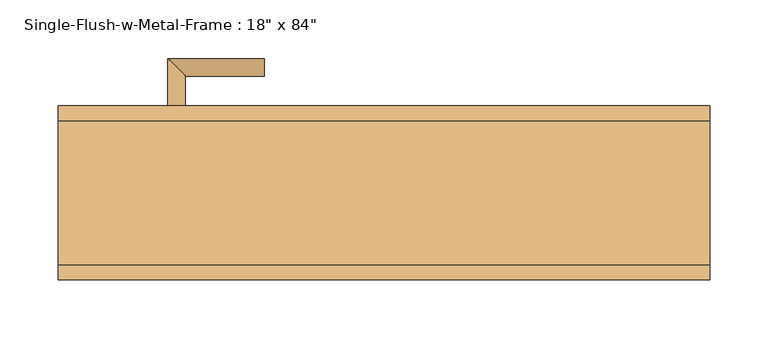
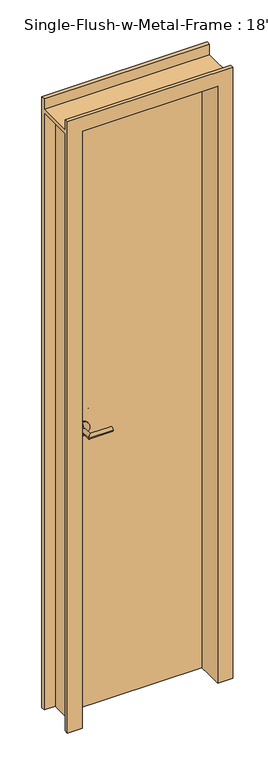
"""IFC4 building model written with IfcOpenShell, lengths in millimetres: door geometry."""

from ifc_helpers import new_model, si_unit, point, frame, origin, origin_with_axes, place, context, project, spatial, polyline, circle_curve, ellipse_curve, trimmed, outline, extrude, faceted_brep, source, transform, mapped, element, save
from ifc_brep_helpers import plane_surface, cylinder_surface, revolved_surface, advanced_brep


def door_d799fe97(model_context):
    return source(origin(), model_context, "Body", "SolidModel", [
        advanced_brep(
        [(-177.8, 14.2875, 971.55), (-177.8, 5.7988821, 989.45), (-185.3, 5.7988821, 996.95), (-177.8, 5.7988821, 1004.45), (-177.8, 14.2875, 1022.35), (-170.3, 5.7988821, 996.95), (-177.8, 17.4625, 1022.35), (-177.8, 17.4625, 971.55), (-177.8, 17.4625, 996.95), (-185.3, -36.1375, 996.95), (-170.3, -21.1375, 996.95), (-102.8, -36.1375, 996.95), (-102.8, -21.1375, 996.95)],
        [
            (0, 1, circle_curve(frame((-177.8, -22.3167775, 965.1541113), z_axis=(1.0, 0.0, 0.0), x_axis=(0.0, 0.0, 1.0)), 37.1588553)),
            (1, 2, circle_curve(frame((-177.8, 5.7988821, 996.95), z_axis=(0.0, 1.0, 0.0), x_axis=(0.0, 0.0, 1.0)), 7.5)),
            (2, 3, circle_curve(frame((-177.8, 5.7988821, 996.95), z_axis=(0.0, 1.0, 0.0), x_axis=(0.0, 0.0, 1.0)), 7.5)),
            (3, 4, circle_curve(frame((-177.8, -22.3167775, 1028.7458887), z_axis=(1.0, 0.0, 0.0), x_axis=(0.0, 0.0, -1.0)), 37.1588553)),
            (4, 0, circle_curve(frame((-177.8, 14.2875, 996.95), z_axis=(0.0, -1.0, 0.0), x_axis=(0.0, 0.0, 1.0)), 25.4)),
            (3, 5, circle_curve(frame((-177.8, 5.7988821, 996.95), z_axis=(0.0, 1.0, 0.0), x_axis=(0.0, 0.0, 1.0)), 7.5)),
            (5, 1, circle_curve(frame((-177.8, 5.7988821, 996.95), z_axis=(0.0, 1.0, 0.0), x_axis=(0.0, 0.0, 1.0)), 7.5)),
            (0, 4, circle_curve(frame((-177.8, 14.2875, 996.95), z_axis=(0.0, -1.0, 0.0), x_axis=(0.0, 0.0, 1.0)), 25.4)),
            (4, 6),
            (6, 7, circle_curve(frame((-177.8, 17.4625, 996.95), z_axis=(0.0, -1.0, 0.0), x_axis=(0.0, 0.0, 1.0)), 25.4)),
            (7, 0),
            (7, 6, circle_curve(frame((-177.8, 17.4625, 996.95), z_axis=(0.0, -1.0, 0.0), x_axis=(0.0, 0.0, 1.0)), 25.4)),
            (6, 8),
            (8, 7),
            (9, 2),
            (5, 10),
            (10, 9, ellipse_curve(frame((-177.8, -28.6375, 996.95), z_axis=(-0.7071067811864695, 0.7071067811866254, 0.0), x_axis=(0.7071067811866254, 0.7071067811864696, 0.0)), 10.6066017, 7.5)),
            (9, 10, ellipse_curve(frame((-177.8, -28.6375, 996.95), z_axis=(-0.7071067811864695, 0.7071067811866254, 0.0), x_axis=(0.7071067811866254, 0.7071067811864696, 0.0)), 10.6066017, 7.5)),
            (11, 12, circle_curve(frame((-102.8, -28.6375, 996.95), z_axis=(1.0, 0.0, 0.0), x_axis=(0.0, 1.0, 0.0)), 7.5)),
            (12, 11, circle_curve(frame((-102.8, -28.6375, 996.95), z_axis=(1.0, 0.0, 0.0), x_axis=(0.0, 1.0, 0.0)), 7.5)),
            (10, 12),
            (11, 9),
        ],
        [
            revolved_surface(trimmed(ellipse_curve(frame((-177.8, -22.3167775, 1028.7458887), z_axis=(1.0, 0.0, 0.0), x_axis=(0.0, 0.0, -1.0)), 37.1588553, 37.1588553), [point((-177.8, 4.7625, 1003.3))], [point((-177.8, 14.2875, 1022.35))], True, "CARTESIAN"), (-177.8, 4.7625, 996.95), (0.0, 1.0, 0.0)),
            cylinder_surface(frame((-177.8, 4.7625, 996.95), z_axis=(0.0, 1.0, 0.0), x_axis=(0.0, 0.0, 1.0)), 25.4),
            plane_surface(frame((-177.8, 17.4625, 996.95), z_axis=(0.0, 1.0, 0.0), x_axis=(0.0, 0.0, 1.0))),
            cylinder_surface(frame((-177.8, 9.4625, 996.95), z_axis=(0.0, 1.0, 0.0), x_axis=(1.0, 0.0, 0.0)), 7.5),
            plane_surface(frame((-102.8, -28.6375, 996.95), z_axis=(1.0, 0.0, 0.0), x_axis=(0.0, 0.0, 1.0))),
            cylinder_surface(frame((-177.8, -28.6375, 996.95), z_axis=(-1.0, 0.0, 0.0), x_axis=(0.0, 1.0, 0.0)), 7.5),
        ],
        [
            (0, [[1, 2, 3, 4, 5]]),
            (0, [[-4, 6, 7, -1, 8]]),
            (1, [[9, 10, 11, -5]]),
            (1, [[-11, 12, -9, -8]]),
            (2, [[13, 14, -10]]),
            (2, [[-14, -13, -12]]),
            (3, [[15, -2, -7, 16, 17]]),
            (3, [[-16, -6, -3, -15, 18]]),
            (4, [[19, 20]]),
            (5, [[21, -19, 22, -17]]),
            (5, [[-22, -20, -21, -18]]),
        ],
    ),
        advanced_brep(
        [(-177.8, 65.0875, 971.55), (-177.8, 65.0875, 1022.35), (-177.8, 73.5761179, 1004.45), (-185.3, 73.5761179, 996.95), (-177.8, 73.5761179, 989.45), (-170.3, 73.5761179, 996.95), (-177.8, 61.9125, 971.55), (-177.8, 61.9125, 1022.35), (-177.8, 61.9125, 996.95), (-185.3, 115.5125, 996.95), (-170.3, 100.5125, 996.95), (-102.8, 115.5125, 996.95), (-102.8, 100.5125, 996.95)],
        [
            (0, 1, circle_curve(frame((-177.8, 65.0875, 996.95), z_axis=(0.0, 1.0, 0.0), x_axis=(0.0, 0.0, 1.0)), 25.4)),
            (1, 2, circle_curve(frame((-177.8, 101.6917775, 1028.7458887), z_axis=(1.0, 0.0, 0.0), x_axis=(0.0, 0.0, -1.0)), 37.1588553)),
            (2, 3, circle_curve(frame((-177.8, 73.5761179, 996.95), z_axis=(0.0, -1.0, 0.0), x_axis=(0.0, 0.0, 1.0)), 7.5)),
            (3, 4, circle_curve(frame((-177.8, 73.5761179, 996.95), z_axis=(0.0, -1.0, 0.0), x_axis=(0.0, 0.0, 1.0)), 7.5)),
            (4, 0, circle_curve(frame((-177.8, 101.6917775, 965.1541113), z_axis=(1.0, 0.0, 0.0), x_axis=(0.0, 0.0, 1.0)), 37.1588553)),
            (1, 0, circle_curve(frame((-177.8, 65.0875, 996.95), z_axis=(0.0, 1.0, 0.0), x_axis=(0.0, 0.0, 1.0)), 25.4)),
            (4, 5, circle_curve(frame((-177.8, 73.5761179, 996.95), z_axis=(0.0, -1.0, 0.0), x_axis=(0.0, 0.0, 1.0)), 7.5)),
            (5, 2, circle_curve(frame((-177.8, 73.5761179, 996.95), z_axis=(0.0, -1.0, 0.0), x_axis=(0.0, 0.0, 1.0)), 7.5)),
            (0, 6),
            (6, 7, circle_curve(frame((-177.8, 61.9125, 996.95), z_axis=(0.0, 1.0, 0.0), x_axis=(0.0, 0.0, 1.0)), 25.4)),
            (7, 1),
            (7, 6, circle_curve(frame((-177.8, 61.9125, 996.95), z_axis=(0.0, 1.0, 0.0), x_axis=(0.0, 0.0, 1.0)), 25.4)),
            (6, 8),
            (8, 7),
            (9, 10, ellipse_curve(frame((-177.8, 108.0125, 996.95), z_axis=(-0.7071067811864695, -0.7071067811866254, 0.0), x_axis=(0.7071067811866254, -0.7071067811864696, 0.0)), 10.6066017, 7.5)),
            (10, 5),
            (3, 9),
            (10, 9, ellipse_curve(frame((-177.8, 108.0125, 996.95), z_axis=(-0.7071067811864695, -0.7071067811866254, 0.0), x_axis=(0.7071067811866254, -0.7071067811864696, 0.0)), 10.6066017, 7.5)),
            (11, 12, circle_curve(frame((-102.8, 108.0125, 996.95), z_axis=(1.0, 0.0, 0.0), x_axis=(0.0, -1.0, 0.0)), 7.5)),
            (12, 11, circle_curve(frame((-102.8, 108.0125, 996.95), z_axis=(1.0, 0.0, 0.0), x_axis=(0.0, -1.0, 0.0)), 7.5)),
            (9, 11),
            (12, 10),
        ],
        [
            revolved_surface(trimmed(ellipse_curve(frame((-177.8, 101.6917775, 1028.7458887), z_axis=(-1.0, 0.0, 0.0), x_axis=(0.0, 0.0, -1.0)), 37.1588553, 37.1588553), [point((-177.8, 74.6125, 1003.3))], [point((-177.8, 65.0875, 1022.35))], True, "CARTESIAN"), (-177.8, 74.6125, 996.95), (0.0, -1.0, 0.0)),
            cylinder_surface(frame((-177.8, 74.6125, 996.95), z_axis=(0.0, -1.0, 0.0), x_axis=(0.0, 0.0, 1.0)), 25.4),
            plane_surface(frame((-177.8, 61.9125, 996.95), z_axis=(0.0, -1.0, 0.0), x_axis=(0.0, 0.0, 1.0))),
            cylinder_surface(frame((-177.8, 69.9125, 996.95), z_axis=(0.0, -1.0, 0.0), x_axis=(1.0, 0.0, 0.0)), 7.5),
            plane_surface(frame((-102.8, 108.0125, 996.95), z_axis=(1.0, 0.0, 0.0), x_axis=(0.0, 0.0, 1.0))),
            cylinder_surface(frame((-177.8, 108.0125, 996.95), z_axis=(-1.0, 0.0, 0.0), x_axis=(0.0, -1.0, 0.0)), 7.5),
        ],
        [
            (0, [[1, 2, 3, 4, 5]]),
            (0, [[6, -5, 7, 8, -2]]),
            (1, [[-1, 9, 10, 11]]),
            (1, [[-6, -11, 12, -9]]),
            (2, [[-10, 13, 14]]),
            (2, [[-12, -14, -13]]),
            (3, [[15, 16, -7, -4, 17]]),
            (3, [[18, -17, -3, -8, -16]]),
            (4, [[19, 20]]),
            (5, [[-15, 21, -20, 22]]),
            (5, [[-18, -22, -19, -21]]),
        ],
    ),
        extrude(outline(polyline([(228.6, 17.4625), (-228.6, 17.4625), (-228.6, 61.9125), (228.6, 61.9125), (228.6, 17.4625)])), origin_with_axes(), (0.0, 0.0, 1.0), 2133.6),
        faceted_brep([(-241.3, 61.9125, 0.0), (-279.4, 61.9125, 0.0), (-279.4, 74.6125, 0.0), (-228.6, 74.6125, 0.0), (-228.6, -74.6125, 0.0), (-279.4, -74.6125, 0.0), (-279.4, -61.9125, 0.0), (-241.3, -61.9125, 0.0), (-241.3, 61.9125, 2133.6), (-279.4, 61.9125, 2133.6), (-279.4, -61.9125, 2133.6), (-279.4, -74.6125, 2184.4), (-279.4, -61.9125, 2184.4), (-279.4, -61.9125, 2146.3), (-279.4, 61.9125, 2146.3), (-279.4, 61.9125, 2184.4), (-279.4, 74.6125, 2184.4), (279.4, 74.6125, 2184.4), (279.4, 74.6125, 0.0), (228.6, 74.6125, 0.0), (228.6, 74.6125, 2133.6), (-228.6, 74.6125, 2133.6), (-228.6, -74.6125, 2133.6), (228.6, -74.6125, 2133.6), (228.6, -74.6125, 0.0), (279.4, -74.6125, 0.0), (279.4, -74.6125, 2184.4), (-241.3, -61.9125, 2133.6), (241.3, 61.9125, 0.0), (241.3, -61.9125, 0.0), (279.4, -61.9125, 0.0), (279.4, 61.9125, 0.0), (279.4, -61.9125, 2146.3), (279.4, -61.9125, 2184.4), (279.4, -61.9125, 2133.6), (279.4, 61.9125, 2133.6), (279.4, 61.9125, 2184.4), (279.4, 61.9125, 2146.3), (241.3, -61.9125, 2133.6), (241.3, 61.9125, 2133.6)], [[[0, 1, 2, 3, 4, 5, 6, 7]], [[1, 0, 8, 9]], [[2, 1, 9, 10, 6, 5, 11, 12, 13, 14, 15, 16]], [[3, 2, 16, 17, 18, 19, 20, 21]], [[4, 3, 21, 22]], [[5, 4, 22, 23, 24, 25, 26, 11]], [[7, 6, 10, 27]], [[0, 7, 27, 8]], [[19, 24, 23, 20]], [[28, 29, 30, 25, 24, 19, 18, 31]], [[32, 33, 26, 25, 30, 34, 35, 31, 18, 17, 36, 37]], [[30, 29, 38, 34]], [[28, 31, 35, 39]], [[29, 28, 39, 38]], [[33, 32, 13, 12]], [[26, 33, 12, 11]], [[10, 9, 8, 27]], [[22, 21, 20, 23]], [[35, 34, 38, 39]], [[36, 17, 16, 15]], [[37, 36, 15, 14]], [[32, 37, 14, 13]]]),
    ])


if __name__ == "__main__":
    model = new_model("IFC4")
    model_context = context("Model", 3, world=origin())
    ifc_project = project(units=[si_unit("LENGTHUNIT", "METRE", prefix="MILLI")], contexts=[model_context])
    site = spatial("IfcSite", under=ifc_project)
    building = spatial("IfcBuilding", under=site)
    placement = place(None, origin())
    door_shape = door_d799fe97(model_context)
    element("IfcDoor", 1, ObjectType="Single-Flush-w-Metal-Frame : 18\" x 84\"", at=placement, inside=building, context=model_context, shape_type="MappedRepresentation", body=[
        mapped(door_shape, transform((0.0, 0.0, 0.0), x_axis=(1.0, 0.0, 0.0), y_axis=(0.0, 1.0, 0.0), z_axis=(0.0, 0.0, 1.0))),
    ])
    save(model, "model.ifc")

# Revit data of these elements
# Type "Single-Flush-w-Metal-Frame : 18\" x 84\""
#   Type Mark = "66"
#   Construction Type Id = "MDOOR"
#   Assembly Code = "C1020"
#   Analytic Construction = "Metal"
#   Thickness = 0' - 1 3/4"
#   Thermal Resistance (R) = 1.5338 (h·ft²·°F)/BTU
#   Half Width Neg = -0' - 11"
#   Half Width = 0' - 11"
#   Frame Width = 0' - 2"
#   Frame Thickness = 0' - 0 1/2"
#   Frame Head Height = 0' - 2"
#   Heat Transfer Coefficient (U) = 0.651978 BTU/(h·ft²·°F)
#   Height = 7' - 0"
#   Width = 1' - 6"
#   Define Thermal Properties by = 1
#   Define Thermal Properties by = 1
#   Door Material = Door - Panel
#   Frame Material = Door - Frame
#   Visual Light Transmittance = 0
#   Solar Heat Gain Coefficient = 0
#   Function = (empty or 0)
#   Wall Closure = (empty or 0)
# Element 1 (IfcDoor, "Single-Flush-w-Metal-Frame : 18\" x 84\"")
#   Materials on its faces: "Metal - Aluminium", "Door - Frame", "Door - Panel"
# Materials
#   "Door - Panel": class "Wood", colour RGB 210 159 95, transparency 0
#   "Door - Frame": class "Miscellaneous", colour RGB 118 70 51, transparency 0
#   "Metal - Aluminium": class "Unassigned", colour RGB 247 247 247, transparency 0
